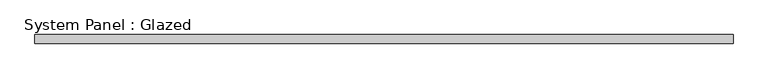
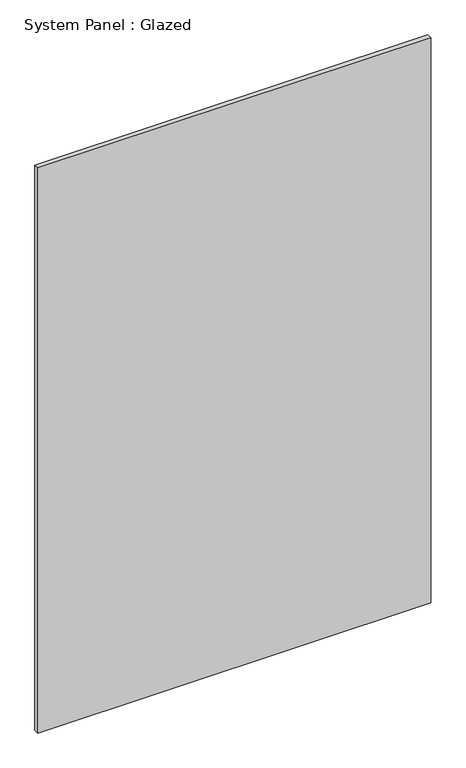
"""IFC4 building model written with IfcOpenShell, lengths in millimetres: plate geometry, System Panel : Glazed."""

from ifc_helpers import new_model, si_unit, origin, origin_with_axes, place, context, project, spatial, polyline, outline, extrude, source, transform, mapped, element, save


def system_panel_glazed_19a6ddb1(model_context):
    return source(origin(), model_context, "Body", "SweptSolid", [
        extrude(outline(polyline([(961.6833335, 24.5), (-961.6833335, 24.5), (-961.6833335, 49.5), (961.6833335, 49.5), (961.6833335, 24.5)])), origin_with_axes(), (0.0, 0.0, 1.0), 2925.0),
    ])


if __name__ == "__main__":
    model = new_model("IFC4")
    model_context = context("Model", 3, world=origin())
    ifc_project = project(units=[si_unit("LENGTHUNIT", "METRE", prefix="MILLI")], contexts=[model_context])
    site = spatial("IfcSite", under=ifc_project)
    building = spatial("IfcBuilding", under=site)
    placement = place(None, origin())
    system_panel_glazed_shape = system_panel_glazed_19a6ddb1(model_context)
    element("IfcPlate", 1, ObjectType="System Panel : Glazed", at=placement, inside=building, context=model_context, shape_type="MappedRepresentation", body=[
        mapped(system_panel_glazed_shape, transform((0.0, 0.0, 0.0), x_axis=(1.0, 0.0, 0.0), y_axis=(0.0, 1.0, 0.0), z_axis=(0.0, 0.0, 1.0))),
    ])
    save(model, "model.ifc")

# Revit data of these elements
# Element 1 (IfcPlate, "System Panel : Glazed")
#   Materials on its faces: "Glass"
# Materials
#   "Glass": class "Glass", colour RGB 0 128 192, transparency 0.9
